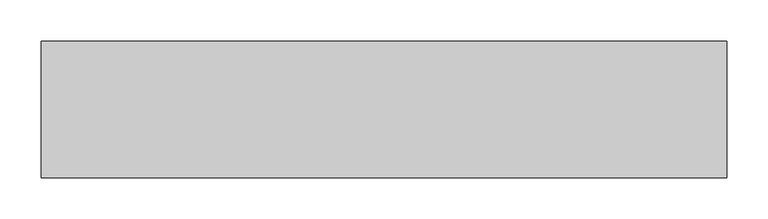
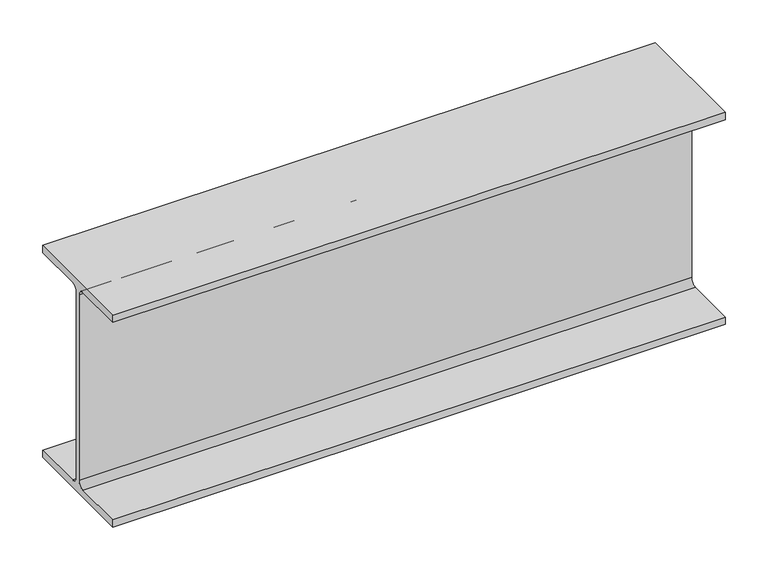
"""IFC4 building model written with IfcOpenShell, lengths in millimetres: beam geometry, Old_Steel Beam_H-KSD3502 : H_SB_ASB_H-390×300x10x16."""

from ifc_helpers import new_model, si_unit, point, frame, frame_2d, origin, place, context, project, spatial, polyline, circle_curve, trimmed, segment, composite_curve, outline, extrude, source, transform, mapped, element, save


def beam_26054666(model_context):
    return source(origin(), model_context, "Body", "SweptSolid", [
        extrude(outline(composite_curve([segment(polyline([(82.5, -141.5), (82.5, -151.7), (-82.5, -151.7), (-82.5, -141.5), (-11.9, -141.5)]), True, "CONTINUOUS"), segment(trimmed(circle_curve(frame_2d((-11.9, -132.6)), 8.9), [point((-11.9, -141.5))], [point((-3.0, -132.6))], True, "CARTESIAN"), True, "CONTINUOUS"), segment(polyline([(-3.0, -132.6), (-3.0, 132.6)]), True, "CONTINUOUS"), segment(trimmed(circle_curve(frame_2d((-11.9, 132.6)), 8.9), [point((-3.0, 132.6))], [point((-11.9, 141.5))], True, "CARTESIAN"), True, "CONTINUOUS"), segment(polyline([(-11.9, 141.5), (-82.5, 141.5), (-82.5, 151.7), (82.5, 151.7), (82.5, 141.5), (11.9, 141.5)]), True, "CONTINUOUS"), segment(trimmed(circle_curve(frame_2d((11.9, 132.6)), 8.9), [point((11.9, 141.5))], [point((3.0, 132.6))], True, "CARTESIAN"), True, "CONTINUOUS"), segment(polyline([(3.0, 132.6), (3.0, -132.6)]), True, "CONTINUOUS"), segment(trimmed(circle_curve(frame_2d((11.9, -132.6)), 8.9), [point((3.0, -132.6))], [point((11.9, -141.5))], True, "CARTESIAN"), True, "CONTINUOUS"), segment(polyline([(11.9, -141.5), (82.5, -141.5)]), True, "CONTINUOUS")], self_intersect=False)), frame((-415.0, 0.0, 0.0), z_axis=(1.0, 0.0, 0.0), x_axis=(0.0, 1.0, 0.0)), (0.0, 0.0, 1.0), 830.0),
    ])


if __name__ == "__main__":
    model = new_model("IFC4")
    model_context = context("Model", 3, world=origin())
    ifc_project = project(units=[si_unit("LENGTHUNIT", "METRE", prefix="MILLI")], contexts=[model_context])
    site = spatial("IfcSite", under=ifc_project)
    building = spatial("IfcBuilding", under=site)
    placement = place(None, origin())
    beam_shape = beam_26054666(model_context)
    element("IfcBeam", 1, ObjectType="Old_Steel Beam_H-KSD3502 : H_SB_ASB_H-390×300x10x16", at=placement, inside=building, context=model_context, shape_type="MappedRepresentation", body=[
        mapped(beam_shape, transform((0.0, 0.0, 0.0), x_axis=(1.0, 0.0, 0.0), y_axis=(0.0, 1.0, 0.0), z_axis=(0.0, 0.0, 1.0))),
    ])
    save(model, "model.ifc")

# Revit data of these elements
# Type "Old_Steel Beam_H-KSD3502 : H_SB_ASB_H-390×300x10x16"
#   Width = 30.0 cm
#   Web Thickness = 1.0 cm
#   Web Fillet = 2.2 cm
#   Warping Constant = 2517770.0 cm⁶
#   Torsional Moment of Inertia = 94.3867 cm⁴
#   Torsional Modulus = 1.0 cm³
#   Section Area = 136.0 cm²
#   Plastic Modulus weak axis = 733.0 cm³
#   Plastic Modulus strong axis = 2190.0 cm³
#   Perimeter = 1.92 m²/m
#   Nominal Weight = 107.00 kgf/m
#   Moment of Inertia weak axis = 7210.00 cm⁴
#   Moment of Inertia strong axis = 38700.00 cm⁴
#   Height = 39.0 cm
#   Flange Thickness = 1.6 cm
#   Elastic Modulus weak axis = 481.0 cm³
#   Elastic Modulus strong axis = 1980.0 cm³
#   Centroid Vertical = 19.5 cm
#   Centroid Horizontal = 15.0 cm
#   Length [instance default] = 1.5240 m
#   Structural Material [instance default] = Steel, 45-345
#   Assembly Code = ""
# Element 1 (IfcBeam, "Old_Steel Beam_H-KSD3502 : H_SB_ASB_H-390×300x10x16")
#   Structural Material = none
# Materials
#   "Steel, 45-345": class "Metal", colour RGB 189 187 185, transparency 0, Description = "Steel 345 MPa", Cost = 0
